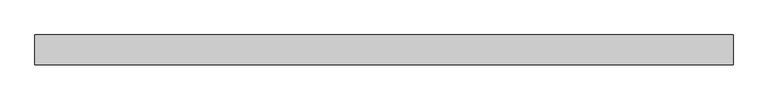
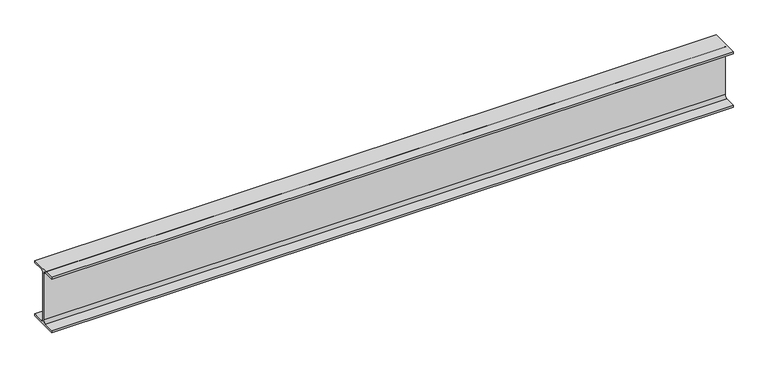
"""IFC4 building model written with IfcOpenShell, lengths in millimetres: beam geometry, 0912_Steel Framing_H-KSD3502 : H_SB_ASB_H-250x125x6x9."""

import ifcopenshell
import ifcopenshell.guid

model = None  # the IFC model being written
_history = None  # IfcOwnerHistory: only IFC2X3 demands one
_inside = {}  # id of a spatial element -> (the spatial element, [elements in it])
_under = {}  # id of a project, library or spatial element -> (it, [spatial elements below it])
_declared = {}  # id of a project -> (the project, [libraries it declares])
_typed = {}  # id of a type object -> (the type object, [elements of that type])
_made_of = {}  # id of a material, layer set ... -> (it, [elements and type objects made of it])


def new_model(schema):
    """Start an empty IFC model of exactly this schema.

    Asked for "IFC4X3", IfcOpenShell would pick the latest addendum, in which some entities
    have other attributes; the version numbers below select the first issue.
    IFC2X3 requires an IfcOwnerHistory on every rooted entity: one is made here for all.
    """
    global model, _history
    if schema == "IFC4X3":
        model = ifcopenshell.file(schema_version=(4, 3, 0, 0))
    else:
        model = ifcopenshell.file(schema=schema)
    _inside.clear()
    _under.clear()
    _declared.clear()
    _typed.clear()
    _made_of.clear()
    _history = None
    if model.schema == "IFC2X3":
        org = make("IfcOrganization", Name="unknown")
        user = make(
            "IfcPersonAndOrganization",
            ThePerson=make("IfcPerson", FamilyName="unknown"),
            TheOrganization=org,
        )
        app = make(
            "IfcApplication",
            ApplicationDeveloper=org,
            Version="unknown",
            ApplicationFullName="unknown",
            ApplicationIdentifier="unknown",
        )
        _history = make(
            "IfcOwnerHistory",
            OwningUser=user,
            OwningApplication=app,
            ChangeAction="ADDED",
            CreationDate=0,
        )
    return model


def make(cls, **values):
    """One entity of the class cls with the attributes given. An attribute that is None is left unset."""
    return model.create_entity(
        cls, **{name: value for name, value in values.items() if value is not None}
    )


def rooted(cls, **values):
    """An entity with a GlobalId (a new one), such as an element, a storey or a relation."""
    return make(cls, GlobalId=ifcopenshell.guid.new(), OwnerHistory=_history, **values)


def si_unit(unit_type, name, prefix=None):
    """IfcSIUnit, for example si_unit("LENGTHUNIT", "METRE", prefix="MILLI")."""
    return make("IfcSIUnit", UnitType=unit_type, Prefix=prefix, Name=name)


def assignment(units):
    """IfcUnitAssignment: the units of a project."""
    return None if units is None else make("IfcUnitAssignment", Units=units)


def point(xyz):
    """IfcCartesianPoint."""
    return None if xyz is None else make("IfcCartesianPoint", Coordinates=xyz)


def direction(xyz):
    """IfcDirection."""
    return None if xyz is None else make("IfcDirection", DirectionRatios=xyz)


def frame(location, z_axis=None, x_axis=None):
    """IfcAxis2Placement3D, a coordinate frame: its origin and axes. An axis left out is left unset."""
    return make(
        "IfcAxis2Placement3D",
        Location=point(location),
        Axis=direction(z_axis),
        RefDirection=direction(x_axis),
    )


def frame_2d(location, x_axis=None):
    """IfcAxis2Placement2D, a coordinate frame in the plane: its origin and x axis."""
    return make(
        "IfcAxis2Placement2D", Location=point(location), RefDirection=direction(x_axis)
    )


def origin():
    """The frame at (0, 0, 0) with its axes left unset."""
    return frame((0.0, 0.0, 0.0))


def place(relative_to, where):
    """IfcLocalPlacement: puts the frame where relative to a parent placement (None: the world)."""
    return make(
        "IfcLocalPlacement", PlacementRelTo=relative_to, RelativePlacement=where
    )


def context(
    kind, dimensions, precision=None, world=None, true_north=None, identifier=None
):
    """IfcGeometricRepresentationContext, for example the 3D "Model" context."""
    return make(
        "IfcGeometricRepresentationContext",
        ContextIdentifier=identifier,
        ContextType=kind,
        CoordinateSpaceDimension=dimensions,
        Precision=precision,
        WorldCoordinateSystem=world,
        TrueNorth=true_north,
    )


def project(units=None, contexts=None):
    """IfcProject with its units and contexts."""
    return rooted(
        "IfcProject",
        Name="project",
        RepresentationContexts=contexts,
        UnitsInContext=assignment(units),
    )


def spatial(cls, under=None, at=None, **own):
    """A site, building, storey or space (cls), placed at a placement, below another one or the project."""
    s = rooted(cls, ObjectPlacement=at, **own)
    if under is not None:
        _under.setdefault(under.id(), (under, []))[1].append(s)
    return s


def polyline(points):
    """IfcPolyline through the points."""
    return make("IfcPolyline", Points=[point(p) for p in points])


def circle_curve(where, radius):
    """IfcCircle in the frame where."""
    return make("IfcCircle", Position=where, Radius=radius)


def trimmed(basis, trim1, trim2, sense, master):
    """IfcTrimmedCurve: the piece of a basis curve between two trims."""
    return make(
        "IfcTrimmedCurve",
        BasisCurve=basis,
        Trim1=trim1,
        Trim2=trim2,
        SenseAgreement=sense,
        MasterRepresentation=master,
    )


def segment(curve, same_sense, transition):
    """IfcCompositeCurveSegment."""
    return make(
        "IfcCompositeCurveSegment",
        Transition=transition,
        SameSense=same_sense,
        ParentCurve=curve,
    )


def composite_curve(segments, self_intersect=None):
    """IfcCompositeCurve: segments joined end to end."""
    return make("IfcCompositeCurve", Segments=segments, SelfIntersect=self_intersect)


def outline(outer, holes=None, kind="AREA"):
    """IfcArbitraryClosedProfileDef: a profile drawn as a closed curve; with holes, ...WithVoids."""
    if holes is None:
        return make("IfcArbitraryClosedProfileDef", ProfileType=kind, OuterCurve=outer)
    return make(
        "IfcArbitraryProfileDefWithVoids",
        ProfileType=kind,
        OuterCurve=outer,
        InnerCurves=holes,
    )


def extrude(swept, where, along, depth):
    """IfcExtrudedAreaSolid: the profile swept, set in the frame where, extruded along a direction by depth."""
    return make(
        "IfcExtrudedAreaSolid",
        SweptArea=swept,
        Position=where,
        ExtrudedDirection=direction(along),
        Depth=depth,
    )


def shape(context_of_items, identifier, shape_type, items):
    """IfcShapeRepresentation: the items that make up one representation, for example the "Body"."""
    return make(
        "IfcShapeRepresentation",
        ContextOfItems=context_of_items,
        RepresentationIdentifier=identifier,
        RepresentationType=shape_type,
        Items=items,
    )


def source(mapping_origin, context_of_items, identifier, shape_type, items):
    """IfcRepresentationMap: a shape defined once, which mapped items show again and again."""
    return make(
        "IfcRepresentationMap",
        MappingOrigin=mapping_origin,
        MappedRepresentation=shape(context_of_items, identifier, shape_type, items),
    )


def transform(
    local_origin,
    x_axis=None,
    y_axis=None,
    z_axis=None,
    scale=None,
    scale2=None,
    scale3=None,
    uniform=True,
):
    """IfcCartesianTransformationOperator3D, or its non-uniform kind. x_axis, y_axis, z_axis: its Axis1, 2, 3."""
    if uniform:
        return make(
            "IfcCartesianTransformationOperator3D",
            Axis1=direction(x_axis),
            Axis2=direction(y_axis),
            LocalOrigin=point(local_origin),
            Scale=scale,
            Axis3=direction(z_axis),
        )
    return make(
        "IfcCartesianTransformationOperator3DnonUniform",
        Axis1=direction(x_axis),
        Axis2=direction(y_axis),
        LocalOrigin=point(local_origin),
        Scale=scale,
        Axis3=direction(z_axis),
        Scale2=scale2,
        Scale3=scale3,
    )


def mapped(mapping_source, mapping_target):
    """IfcMappedItem: shows the shape of a source again, moved by a transform."""
    return make(
        "IfcMappedItem", MappingSource=mapping_source, MappingTarget=mapping_target
    )


def made_of(thing, what):
    """Note that an element or type object is made of a material, layer set ...; save() writes the relation."""
    if what is not None:
        _made_of.setdefault(what.id(), (what, []))[1].append(thing)
    return thing


def element(
    cls,
    number,
    at=None,
    inside=None,
    cuts=None,
    type_object=None,
    material=None,
    context=None,
    identifier="Body",
    shape_type=None,
    held_by="IfcProductDefinitionShape",
    body=None,
    shapes=None,
    **own,
):
    """One element of the class cls, such as IfcWall. Its Tag is "e" and its number.

    at: its placement. inside: the storey or other place that contains it. cuts: it is an
    opening in that element (IfcRelVoidsElement). A single representation is given by context,
    identifier, shape_type and body (its items); several are given by shapes. held_by: the class
    of the entity that holds the representations. save() writes the other relations.
    """
    e = rooted(cls, Tag="e%d" % number, ObjectPlacement=at, **own)
    if body is not None:
        shapes = [shape(context, identifier, shape_type, body)]
    if shapes is not None:
        e.Representation = make(held_by, Representations=shapes)
    if inside is not None:
        _inside.setdefault(inside.id(), (inside, []))[1].append(e)
    if cuts is not None:
        rooted(
            "IfcRelVoidsElement", RelatingBuildingElement=cuts, RelatedOpeningElement=e
        )
    if type_object is not None:
        _typed.setdefault(type_object.id(), (type_object, []))[1].append(e)
    return made_of(e, material)


def aggregate(whole, parts):
    """IfcRelAggregates: a whole, such as a stair, and the parts it consists of."""
    return rooted("IfcRelAggregates", RelatingObject=whole, RelatedObjects=parts)


def save(model, path):
    """Write the relations noted so far, then the file.

    IfcRelAggregates (storeys below a building ...), IfcRelContainedInSpatialStructure (elements
    in a storey), IfcRelDefinesByType, IfcRelAssociatesMaterial and IfcRelDeclares: one each for
    every whole, place, type object, material and project.
    """
    for whole, parts in _under.values():
        aggregate(whole, parts)
    for where, things in _inside.values():
        rooted(
            "IfcRelContainedInSpatialStructure",
            RelatedElements=things,
            RelatingStructure=where,
        )
    for kind, things in _typed.values():
        rooted("IfcRelDefinesByType", RelatedObjects=things, RelatingType=kind)
    for what, things in _made_of.values():
        rooted("IfcRelAssociatesMaterial", RelatedObjects=things, RelatingMaterial=what)
    for by, libraries in _declared.values():
        rooted("IfcRelDeclares", RelatingContext=by, RelatedDefinitions=libraries)
    model.write(path)


def beam_ab81005f(model_context):
    return source(origin(), model_context, "Body", "SweptSolid", [
        extrude(outline(composite_curve([segment(polyline([(62.5, -116.0), (62.5, -125.0), (-62.5, -125.0), (-62.5, -116.0), (-15.0, -116.0)]), True, "CONTINUOUS"), segment(trimmed(circle_curve(frame_2d((-15.0, -104.0)), 12.0), [point((-15.0, -116.0))], [point((-3.0, -104.0))], True, "CARTESIAN"), True, "CONTINUOUS"), segment(polyline([(-3.0, -104.0), (-3.0, 104.0)]), True, "CONTINUOUS"), segment(trimmed(circle_curve(frame_2d((-15.0, 104.0)), 12.0), [point((-3.0, 104.0))], [point((-15.0, 116.0))], True, "CARTESIAN"), True, "CONTINUOUS"), segment(polyline([(-15.0, 116.0), (-62.5, 116.0), (-62.5, 125.0), (62.5, 125.0), (62.5, 116.0), (15.0, 116.0)]), True, "CONTINUOUS"), segment(trimmed(circle_curve(frame_2d((15.0, 104.0)), 12.0), [point((15.0, 116.0))], [point((3.0, 104.0))], True, "CARTESIAN"), True, "CONTINUOUS"), segment(polyline([(3.0, 104.0), (3.0, -104.0)]), True, "CONTINUOUS"), segment(trimmed(circle_curve(frame_2d((15.0, -104.0)), 12.0), [point((3.0, -104.0))], [point((15.0, -116.0))], True, "CARTESIAN"), True, "CONTINUOUS"), segment(polyline([(15.0, -116.0), (62.5, -116.0)]), True, "CONTINUOUS")], self_intersect=False)), frame((-1529.8000466, 0.0, 0.0), z_axis=(1.0, 0.0, 0.0), x_axis=(0.0, 1.0, 0.0)), (0.0, 0.0, 1.0), 2912.0982036),
    ])


if __name__ == "__main__":
    model = new_model("IFC4")
    model_context = context("Model", 3, world=origin())
    ifc_project = project(units=[si_unit("LENGTHUNIT", "METRE", prefix="MILLI")], contexts=[model_context])
    site = spatial("IfcSite", under=ifc_project)
    building = spatial("IfcBuilding", under=site)
    placement = place(None, origin())
    beam_shape = beam_ab81005f(model_context)
    element("IfcBeam", 1, ObjectType="0912_Steel Framing_H-KSD3502 : H_SB_ASB_H-250x125x6x9", at=placement, inside=building, context=model_context, shape_type="MappedRepresentation", body=[
        mapped(beam_shape, transform((0.0, 0.0, 0.0), x_axis=(1.0, 0.0, 0.0), y_axis=(0.0, 1.0, 0.0), z_axis=(0.0, 0.0, 1.0))),
    ])
    save(model, "model.ifc")

# Revit data of these elements
# Type "0912_Steel Framing_H-KSD3502 : H_SB_ASB_H-250x125x6x9"
#   H_WM Code_1 = "S01AA003-00001 | Main Steel Structure Fabrication Work | Shelter/Building | Light Steel - Standard (30KG/M>Weight) | Material: (   )"
#   H_WM Code_2 = "S03AA029-00001 | Main Steel Structure Erection Work | Shelter/Building | Light Steel (30KG/M>Weight) | Material: (   )"
#   H_WM Code_3 = "S01AA010-00001 | Main Steel Structure Fabrication Work | Shelter/Building | Steel Painting/Coating | for Non-Fireproofed Steel Surface, Surface Preparation, Primer, Second & Final Coat | Material: (   )"
#   H_Q'ty Cal Type Tag = "SB-Q2"
#   Width = 12.5 cm
#   Web Thickness = 0.6 cm
#   Web Fillet = 1.2 cm
#   Warping Constant = 42539.8 cm⁶
#   W = 0
#   Torsional Moment of Inertia = 7.8102 cm⁴
#   Section Area = 37.66 cm²
#   Plastic Modulus weak axis = 73.1 cm³
#   Plastic Modulus strong axis = 366.0 cm³
#   Perimeter = 0.97 m²/m
#   Nominal Weight = 29.60 kgf/m
#   Moment of Inertia weak axis = 294.00 cm⁴
#   Moment of Inertia strong axis = 4050.00 cm⁴
#   Height = 25.0 cm
#   Flange Thickness = 0.9 cm
#   Elastic Modulus weak axis = 47.0 cm³
#   Elastic Modulus strong axis = 324.0 cm³
#   Centroid Vertical = 12.5 cm
#   Centroid Horizontal = 6.25 cm
#   Ix = 40500000
#   Length [instance default] = 1.5240 m
#   Zx = 366000
#   b = 0.1250 m
#   h = 0.2500 m
#   r = 0.0120 m
#   s = 0.0060 m
#   t = 0.0090 m
#   A = 0.003766 m²
#   Structural Material [instance default] = Steel, 45-345
#   Assembly Code = ""
# Element 1 (IfcBeam, "0912_Steel Framing_H-KSD3502 : H_SB_ASB_H-250x125x6x9")
#   Structural Material = none
# Materials
#   "Steel, 45-345": class "Metal", colour RGB 189 187 185, transparency 0, Description = "Steel 345 MPa", Cost = 0
